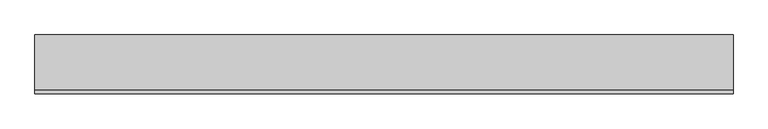
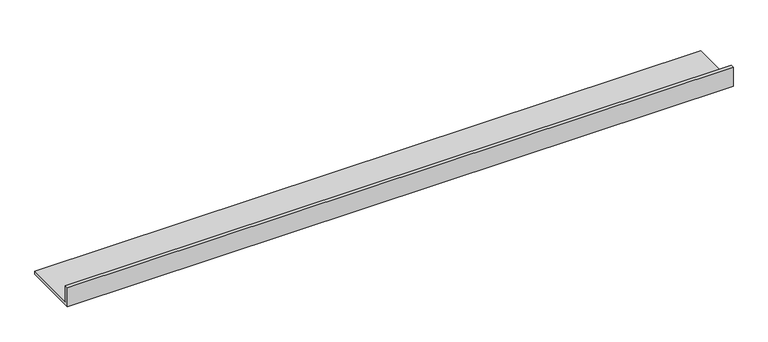
"""IFC4 building model written with IfcOpenShell, lengths in millimetres: proxy geometry, 거터2 : 거터2."""

from ifc_helpers import new_model, si_unit, frame, origin, place, context, project, spatial, polyline, outline, extrude, source, transform, mapped, element, save


def generic_models_b95aee2c(model_context):
    return source(origin(), model_context, "Body", "SweptSolid", [
        extrude(outline(polyline([(38999.5208589, 6299.9720055), (38999.5208589, 6599.2986846), (39049.5208589, 6599.2986846), (39049.5208589, 6349.9720055), (39839.5208589, 6349.9720055), (39839.5208589, 6299.9720055), (38999.5208589, 6299.9720055)])), frame((40675.0, 0.0, 0.0), z_axis=(1.0, 0.0, 0.0), x_axis=(0.0, 1.0, 0.0)), (0.0, 0.0, 1.0), 9925.0),
    ])


if __name__ == "__main__":
    model = new_model("IFC4")
    model_context = context("Model", 3, world=origin())
    ifc_project = project(units=[si_unit("LENGTHUNIT", "METRE", prefix="MILLI")], contexts=[model_context])
    site = spatial("IfcSite", under=ifc_project)
    building = spatial("IfcBuilding", under=site)
    placement = place(None, origin())
    generic_models_shape = generic_models_b95aee2c(model_context)
    element("IfcBuildingElementProxy", 1, Name="거터2 : 거터2", ObjectType="거터2 : 거터2", at=placement, inside=building, context=model_context, shape_type="MappedRepresentation", body=[
        mapped(generic_models_shape, transform((0.0, 0.0, 0.0), x_axis=(1.0, 0.0, 0.0), y_axis=(0.0, 1.0, 0.0), z_axis=(0.0, 0.0, 1.0))),
    ])
    save(model, "model.ifc")
